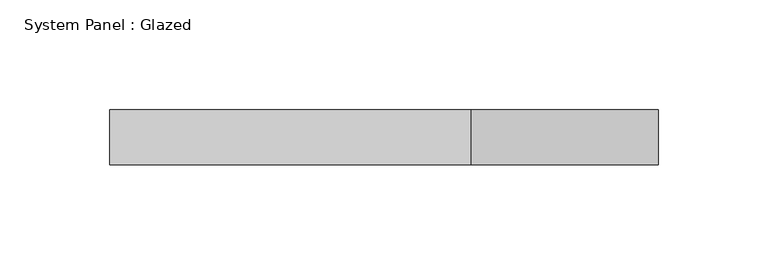
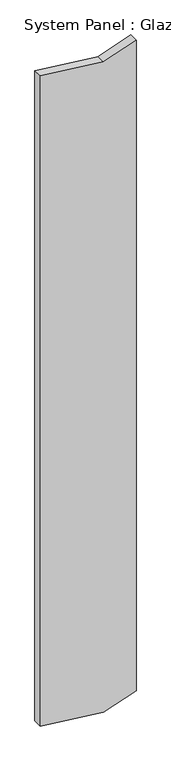
"""IFC4 building model written with IfcOpenShell, lengths in millimetres: plate geometry, System Panel : Glazed."""

from ifc_helpers import new_model, si_unit, frame, origin, place, context, project, spatial, polyline, outline, extrude, source, transform, mapped, element, save


def system_panel_glazed_1952c682(model_context):
    return source(origin(), model_context, "Body", "SweptSolid", [
        extrude(outline(polyline([(18.994214, -125.0), (0.0, 39.6668968), (29.9265022, 125.0), (1826.842902, 125.0), (1796.9625606, 39.7989266), (1815.9726112, -125.0), (18.994214, -125.0)])), frame((0.0, -49.5, 0.0), z_axis=(0.0, 1.0, 0.0), x_axis=(0.0, 0.0, 1.0)), (0.0, 0.0, 1.0), 25.0),
    ])


if __name__ == "__main__":
    model = new_model("IFC4")
    model_context = context("Model", 3, world=origin())
    ifc_project = project(units=[si_unit("LENGTHUNIT", "METRE", prefix="MILLI")], contexts=[model_context])
    site = spatial("IfcSite", under=ifc_project)
    building = spatial("IfcBuilding", under=site)
    placement = place(None, origin())
    system_panel_glazed_shape = system_panel_glazed_1952c682(model_context)
    element("IfcPlate", 1, ObjectType="System Panel : Glazed", at=placement, inside=building, context=model_context, shape_type="MappedRepresentation", body=[
        mapped(system_panel_glazed_shape, transform((0.0, 0.0, 0.0), x_axis=(1.0, 0.0, 0.0), y_axis=(0.0, 1.0, 0.0), z_axis=(0.0, 0.0, 1.0))),
    ])
    save(model, "model.ifc")

# Revit data of these elements
# Element 1 (IfcPlate, "System Panel : Glazed")
#   Materials on its faces: "Glass"
# Materials
#   "Glass": class "Glass", colour RGB 218 227 224, transparency 0.85, Description = "Soda Lime Glass", Cost = 0
